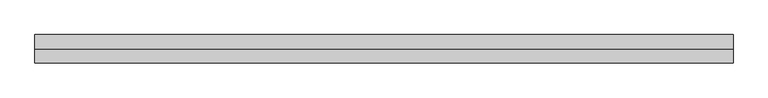
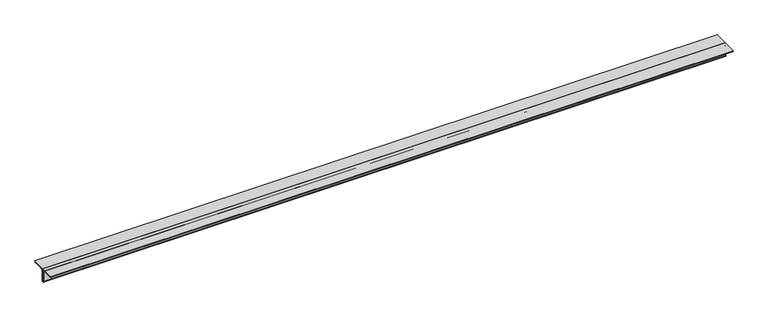
"""IFC4 building model written with IfcOpenShell, lengths in millimetres: member geometry, Steel Framing_2Ls_KS : H_SB_AR_S02_2Ls-100x100x10_VBR1."""

from ifc_helpers import new_model, si_unit, point, frame, frame_2d, origin, place, context, project, spatial, polyline, circle_curve, trimmed, segment, composite_curve, outline, extrude, source, transform, mapped, element, save


def member_ef8e9ece(model_context):
    return source(origin(), model_context, "Body", "SweptSolid", [
        extrude(outline(composite_curve([segment(polyline([(0.0, 28.2), (100.0, 28.2)]), True, "CONTINUOUS"), segment(trimmed(circle_curve(frame_2d((90.0, 28.2)), 10.0), [point((100.0, 28.2))], [point((90.0, 18.2))], False, "CARTESIAN"), True, "CONTINUOUS"), segment(polyline([(90.0, 18.2), (20.0, 18.2)]), True, "CONTINUOUS"), segment(trimmed(circle_curve(frame_2d((20.0, 8.2)), 10.0), [point((20.0, 18.2))], [point((10.0, 8.2))], True, "CARTESIAN"), True, "CONTINUOUS"), segment(polyline([(10.0, 8.2), (10.0, -61.8)]), True, "CONTINUOUS"), segment(trimmed(circle_curve(frame_2d((0.0, -61.8)), 10.0), [point((10.0, -61.8))], [point((0.0, -71.8))], False, "CARTESIAN"), True, "CONTINUOUS"), segment(polyline([(0.0, -71.8), (0.0, 28.2)]), True, "CONTINUOUS")], self_intersect=False)), frame((-2164.6759951, 0.0, 0.0), z_axis=(1.0, 0.0, 0.0), x_axis=(0.0, 1.0, 0.0)), (0.0, 0.0, 1.0), 4915.1757569),
        extrude(outline(composite_curve([segment(polyline([(0.0, 28.2), (0.0, -71.8)]), True, "CONTINUOUS"), segment(trimmed(circle_curve(frame_2d((0.0, -61.8)), 10.0), [point((0.0, -71.8))], [point((-10.0, -61.8))], False, "CARTESIAN"), True, "CONTINUOUS"), segment(polyline([(-10.0, -61.8), (-10.0, 8.2)]), True, "CONTINUOUS"), segment(trimmed(circle_curve(frame_2d((-20.0, 8.2)), 10.0), [point((-10.0, 8.2))], [point((-20.0, 18.2))], True, "CARTESIAN"), True, "CONTINUOUS"), segment(polyline([(-20.0, 18.2), (-90.0, 18.2)]), True, "CONTINUOUS"), segment(trimmed(circle_curve(frame_2d((-90.0, 28.2)), 10.0), [point((-90.0, 18.2))], [point((-100.0, 28.2))], False, "CARTESIAN"), True, "CONTINUOUS"), segment(polyline([(-100.0, 28.2), (0.0, 28.2)]), True, "CONTINUOUS")], self_intersect=False)), frame((-2164.6759951, 0.0, 0.0), z_axis=(1.0, 0.0, 0.0), x_axis=(0.0, 1.0, 0.0)), (0.0, 0.0, 1.0), 4915.1757569),
    ])


if __name__ == "__main__":
    model = new_model("IFC4")
    model_context = context("Model", 3, world=origin())
    ifc_project = project(units=[si_unit("LENGTHUNIT", "METRE", prefix="MILLI")], contexts=[model_context])
    site = spatial("IfcSite", under=ifc_project)
    building = spatial("IfcBuilding", under=site)
    placement = place(None, origin())
    member_shape = member_ef8e9ece(model_context)
    element("IfcMember", 1, ObjectType="Steel Framing_2Ls_KS : H_SB_AR_S02_2Ls-100x100x10_VBR1", at=placement, inside=building, context=model_context, shape_type="MappedRepresentation", body=[
        mapped(member_shape, transform((0.0, 0.0, 0.0), x_axis=(1.0, 0.0, 0.0), y_axis=(0.0, 1.0, 0.0), z_axis=(0.0, 0.0, 1.0))),
    ])
    save(model, "model.ifc")

# Revit data of these elements
# Type "Steel Framing_2Ls_KS : H_SB_AR_S02_2Ls-100x100x10_VBR1"
#   Type Comments = "MAIN"
#   Type Mark = "VBR1"
#   H_SectionID = "2Ls-100x100x10"
#   Assembly Code = "B10"
#   Legs = "LLBB"
#   H_Ratio for Additional Steel Plate = 0.2
#   W = 0
#   Perimeter = 0.80 m²/m
#   Nominal Weight = 29.80 kgf/m
#   Length [instance default] = 1524 mm
#   Space = 0 mm
#   b = 100 mm
#   d = 100 mm
#   t = 10 mm
#   y = 28.2 mm
#   A = 0.0038 m²
#   Structural Material [instance default] = Steel, 45-345
# Element 1 (IfcMember, "Steel Framing_2Ls_KS : H_SB_AR_S02_2Ls-100x100x10_VBR1")
#   Materials on its faces: "Steel, 45-345"
# Materials
#   "Steel, 45-345": class "Metal", colour RGB 189 187 185, transparency 0, Description = "Steel 345 MPa", Cost = 0
